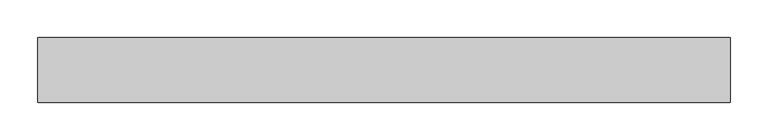
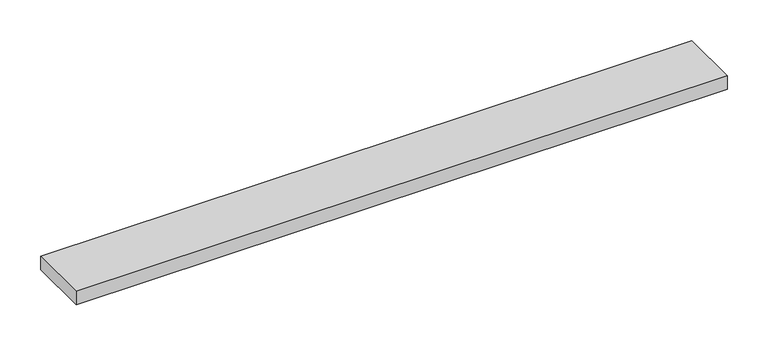
"""IFC4 building model written with IfcOpenShell, lengths in millimetres: proxy geometry, Generic Models 6:Generic Models 2:318829:Generic Models 2:318829 : Generic Models 6:Generic Models 2:318829:13 : Generic Models 6:Generic Models 2:318829:Generic Models 2:318829 : Generic Models 6:Generic Models 2:318829:300683."""

from ifc_helpers import new_model, si_unit, frame, origin, place, context, project, spatial, polyline, outline, extrude, source, transform, mapped, element, save


def generic_models_62d90bf7(model_context):
    return source(origin(), model_context, "Body", "SweptSolid", [
        extrude(outline(polyline([(593679.9536635, -579003.173699), (593679.9536635, -579089.5913841), (592758.9138536, -579089.5913841), (592758.9138536, -579003.173699), (593679.9536635, -579003.173699)])), frame((0.0, 0.0, 3.1263373), z_axis=(0.0, 0.0, 1.0), x_axis=(1.0, 0.0, 0.0)), (0.0, 0.0, 1.0), 20.0608068),
    ])


if __name__ == "__main__":
    model = new_model("IFC4")
    model_context = context("Model", 3, world=origin())
    ifc_project = project(units=[si_unit("LENGTHUNIT", "METRE", prefix="MILLI")], contexts=[model_context])
    site = spatial("IfcSite", under=ifc_project)
    building = spatial("IfcBuilding", under=site)
    placement = place(None, origin())
    generic_models_shape = generic_models_62d90bf7(model_context)
    element("IfcBuildingElementProxy", 1, Name="Generic Models 6:Generic Models 2:318829:Generic Models 2:318829 : Generic Models 6:Generic Models 2:318829:13 : Generic Models 6:Generic Models 2:318829:Generic Models 2:318829 : Generic Models 6:Generic Models 2:318829:300683", ObjectType="Generic Models 6:Generic Models 2:318829:Generic Models 2:318829 : Generic Models 6:Generic Models 2:318829:13 : Generic Models 6:Generic Models 2:318829:Generic Models 2:318829 : Generic Models 6:Generic Models 2:318829:300683", at=placement, inside=building, context=model_context, shape_type="MappedRepresentation", body=[
        mapped(generic_models_shape, transform((0.0, 0.0, 0.0), x_axis=(1.0, 0.0, 0.0), y_axis=(0.0, 1.0, 0.0), z_axis=(0.0, 0.0, 1.0))),
    ])
    save(model, "model.ifc")

# Revit data of these elements
# Type "Generic Models 6:Generic Models 2:318829:Generic Models 2:318829 : Generic Models 6:Generic Models 2:318829:13 : Generic Models 6:Generic Models 2:318829:Generic Models 2:318829 : Generic Models 6:Generic Models 2:318829:300683"
#   NameOverride = "Generic Models 6:Generic Models 2:318829:Generic Models 2:318829 : Generic Models 6:Generic Models 2:318829:300683"
#   ObjectTypeOverride = "Generic Models 2:318829 : Generic Models 6:Generic Models 2:318829"
#   Reference = "Generic Models 2"
#   Tag = "300683"
# Element 1 (IfcBuildingElementProxy, "Generic Models 6:Generic Models 2:318829:Generic Models 2:318829 : Generic Models 6:Generic Models 2:318829:13 : Generic Models 6:Generic Models 2:318829:Generic Models 2:318829 : Generic Models 6:Generic Models 2:318829:300683")
#   Materials on its faces: "PRESSURE TREATED WOOD BLOCKING - SIZE AS NECESSARY"
# Materials
#   "PRESSURE TREATED WOOD BLOCKING - SIZE AS NECESSARY": class "Wood", colour RGB 144 113 62, transparency 0, Description = "Pinus Echinata", Cost = 0
